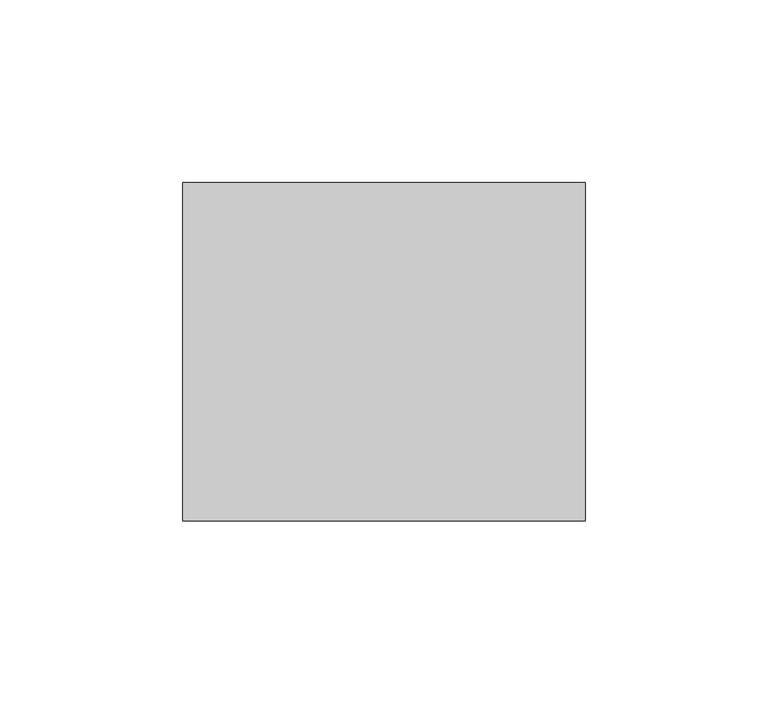
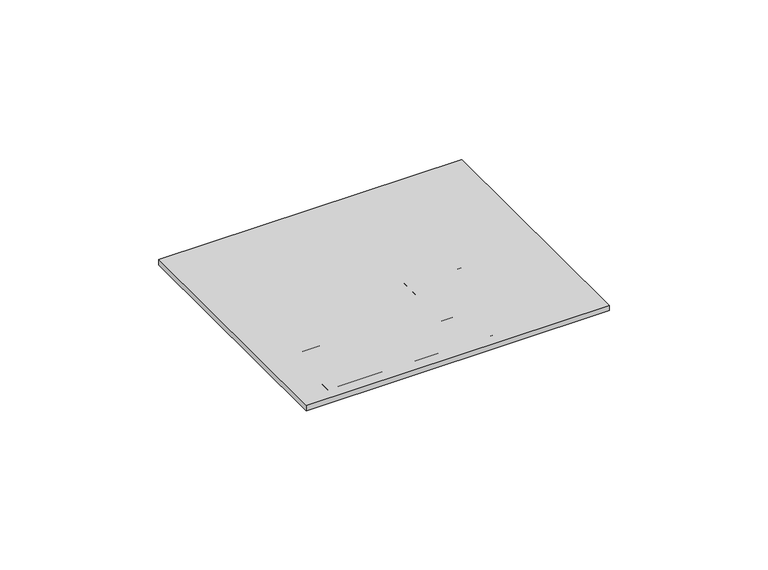
"""IFC4 building model written with IfcOpenShell, lengths in millimetres: proxy geometry, ELE-INTERFONO : VIDEO_PORTERO-Vivienda."""

from ifc_helpers import new_model, si_unit, origin, origin_with_axes, place, context, project, spatial, polyline, outline, extrude, source, transform, mapped, element, save


def electrical_fixtures_7d63f3e9(model_context):
    return source(origin(), model_context, "Body", "SweptSolid", [
        extrude(outline(polyline([(-55.0, 0.0), (55.0, 0.0), (55.0, -92.5), (-55.0, -92.5), (-55.0, 0.0)])), origin_with_axes(), (0.0, 0.0, 1.0), 2.0),
        extrude(outline(polyline([(45.0, -51.8), (5.0, -51.8), (5.0, -48.2), (45.0, -48.2), (45.0, -51.8)])), origin_with_axes(), (0.0, 0.0, 1.0), 2.2),
        extrude(outline(polyline([(45.0, -59.2), (5.0, -59.2), (5.0, -55.6), (45.0, -55.6), (45.0, -59.2)])), origin_with_axes(), (0.0, 0.0, 1.0), 2.2),
        extrude(outline(polyline([(45.0, -74.0), (5.0, -74.0), (5.0, -70.4), (45.0, -70.4), (45.0, -74.0)])), origin_with_axes(), (0.0, 0.0, 1.0), 2.2),
        extrude(outline(polyline([(45.0, -66.6), (5.0, -66.6), (5.0, -63.0), (45.0, -63.0), (45.0, -66.6)])), origin_with_axes(), (0.0, 0.0, 1.0), 2.2),
        extrude(outline(polyline([(45.0, -81.4), (5.0, -81.4), (5.0, -77.8), (45.0, -77.8), (45.0, -81.4)])), origin_with_axes(), (0.0, 0.0, 1.0), 2.2),
        extrude(outline(polyline([(45.0, -88.8), (5.0, -88.8), (5.0, -85.2), (45.0, -85.2), (45.0, -88.8)])), origin_with_axes(), (0.0, 0.0, 1.0), 2.2),
        extrude(outline(polyline([(-45.0, -51.8), (-45.0, -48.2), (-5.0, -48.2), (-5.0, -51.8), (-45.0, -51.8)])), origin_with_axes(), (0.0, 0.0, 1.0), 2.2),
        extrude(outline(polyline([(-45.0, -59.2), (-45.0, -55.6), (-5.0, -55.6), (-5.0, -59.2), (-45.0, -59.2)])), origin_with_axes(), (0.0, 0.0, 1.0), 2.2),
        extrude(outline(polyline([(-45.0, -74.0), (-45.0, -70.4), (-5.0, -70.4), (-5.0, -74.0), (-45.0, -74.0)])), origin_with_axes(), (0.0, 0.0, 1.0), 2.2),
        extrude(outline(polyline([(-45.0, -66.6), (-45.0, -63.0), (-5.0, -63.0), (-5.0, -66.6), (-45.0, -66.6)])), origin_with_axes(), (0.0, 0.0, 1.0), 2.2),
        extrude(outline(polyline([(-45.0, -81.4), (-45.0, -77.8), (-5.0, -77.8), (-5.0, -81.4), (-45.0, -81.4)])), origin_with_axes(), (0.0, 0.0, 1.0), 2.2),
        extrude(outline(polyline([(-45.0, -88.8), (-45.0, -85.2), (-5.0, -85.2), (-5.0, -88.8), (-45.0, -88.8)])), origin_with_axes(), (0.0, 0.0, 1.0), 2.2),
    ])


if __name__ == "__main__":
    model = new_model("IFC4")
    model_context = context("Model", 3, world=origin())
    ifc_project = project(units=[si_unit("LENGTHUNIT", "METRE", prefix="MILLI")], contexts=[model_context])
    site = spatial("IfcSite", under=ifc_project)
    building = spatial("IfcBuilding", under=site)
    placement = place(None, origin())
    electrical_fixtures_shape = electrical_fixtures_7d63f3e9(model_context)
    element("IfcBuildingElementProxy", 1, Name="ELE-INTERFONO : VIDEO_PORTERO-Vivienda", ObjectType="ELE-INTERFONO : VIDEO_PORTERO-Vivienda", at=placement, inside=building, context=model_context, shape_type="MappedRepresentation", body=[
        mapped(electrical_fixtures_shape, transform((0.0, 0.0, 0.0), x_axis=(1.0, 0.0, 0.0), y_axis=(0.0, 1.0, 0.0), z_axis=(0.0, 0.0, 1.0))),
    ])
    save(model, "model.ifc")

# Revit data of these elements
# Type "ELE-INTERFONO : VIDEO_PORTERO-Vivienda"
#   Etiqueta = "I"
#   SímboloPosiciónVertical [instance default] = 0.04 m
#   Anchura = 0.11 m
#   Altura = 0.0925 m
#   Profundidad = 0.0079 m
#   Default Elevation = 0.0014 m
#   SímboloVivienda = yes
#   SímboloPortal = no
#   Material de altavoz = none
